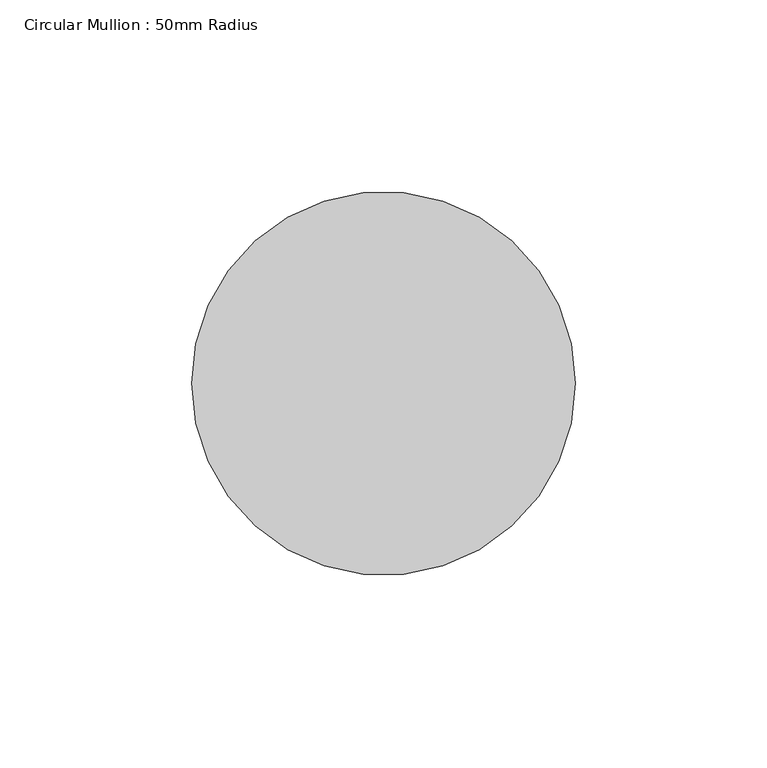
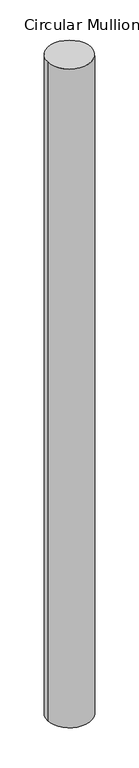
"""IFC4 building model written with IfcOpenShell, lengths in millimetres: member geometry, Circular Mullion : 50mm Radius."""

from ifc_helpers import new_model, si_unit, point, frame, origin, origin_2d, place, context, project, spatial, circle_curve, trimmed, segment, composite_curve, outline, extrude, source, transform, mapped, element, save


def circular_mullion_50mm_radius_2743aa95(model_context):
    return source(origin(), model_context, "Body", "SweptSolid", [
        extrude(outline(composite_curve([segment(trimmed(circle_curve(origin_2d(), 50.0), [point((50.0, 0.0))], [point((-50.0, 0.0))], False, "CARTESIAN"), True, "CONTINUOUS"), segment(trimmed(circle_curve(origin_2d(), 50.0), [point((-50.0, 0.0))], [point((50.0, 0.0))], False, "CARTESIAN"), True, "CONTINUOUS")], self_intersect=False)), frame((0.0, 0.0, -1594.0190235), z_axis=(0.0, 0.0, 1.0), x_axis=(1.0, 0.0, 0.0)), (0.0, 0.0, 1.0), 1594.0190235),
    ])


if __name__ == "__main__":
    model = new_model("IFC4")
    model_context = context("Model", 3, world=origin())
    ifc_project = project(units=[si_unit("LENGTHUNIT", "METRE", prefix="MILLI")], contexts=[model_context])
    site = spatial("IfcSite", under=ifc_project)
    building = spatial("IfcBuilding", under=site)
    placement = place(None, origin())
    circular_mullion_50mm_radius_shape = circular_mullion_50mm_radius_2743aa95(model_context)
    element("IfcMember", 1, ObjectType="Circular Mullion : 50mm Radius", at=placement, inside=building, context=model_context, shape_type="MappedRepresentation", body=[
        mapped(circular_mullion_50mm_radius_shape, transform((0.0, 0.0, 0.0), x_axis=(1.0, 0.0, 0.0), y_axis=(0.0, 1.0, 0.0), z_axis=(0.0, 0.0, 1.0))),
    ])
    save(model, "model.ifc")

# Revit data of these elements
# Type "Circular Mullion : 50mm Radius"
#   built-in parameter 1007350 = 0.164042 (stored number, unit not read)
# Element 1 (IfcMember, "Circular Mullion : 50mm Radius")
#   Materials on its faces: "Aluminium"
# Materials
#   "Aluminium": class "Metal", colour RGB 247 247 247, transparency 0, Description = "Aluminium 6061", Cost = 0
